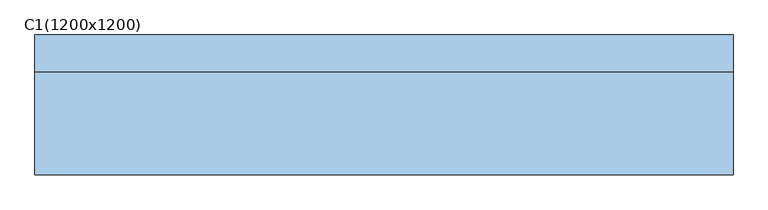
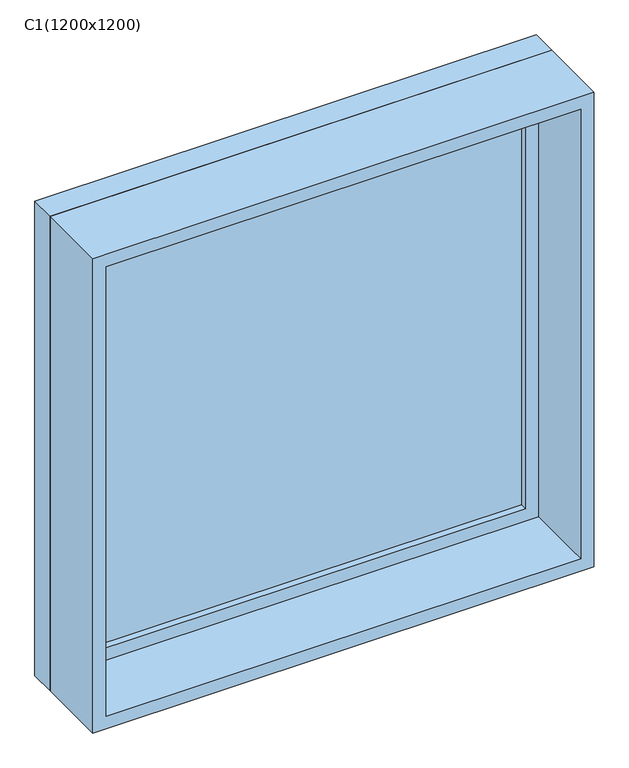
"""IFC4 building model written with IfcOpenShell, lengths in millimetres: window geometry, 固定窗 : C1(1200x1200)."""

import ifcopenshell
import ifcopenshell.guid

model = None  # the IFC model being written
_history = None  # IfcOwnerHistory: only IFC2X3 demands one
_inside = {}  # id of a spatial element -> (the spatial element, [elements in it])
_under = {}  # id of a project, library or spatial element -> (it, [spatial elements below it])
_declared = {}  # id of a project -> (the project, [libraries it declares])
_typed = {}  # id of a type object -> (the type object, [elements of that type])
_made_of = {}  # id of a material, layer set ... -> (it, [elements and type objects made of it])


def new_model(schema):
    """Start an empty IFC model of exactly this schema.

    Asked for "IFC4X3", IfcOpenShell would pick the latest addendum, in which some entities
    have other attributes; the version numbers below select the first issue.
    IFC2X3 requires an IfcOwnerHistory on every rooted entity: one is made here for all.
    """
    global model, _history
    if schema == "IFC4X3":
        model = ifcopenshell.file(schema_version=(4, 3, 0, 0))
    else:
        model = ifcopenshell.file(schema=schema)
    _inside.clear()
    _under.clear()
    _declared.clear()
    _typed.clear()
    _made_of.clear()
    _history = None
    if model.schema == "IFC2X3":
        org = make("IfcOrganization", Name="unknown")
        user = make(
            "IfcPersonAndOrganization",
            ThePerson=make("IfcPerson", FamilyName="unknown"),
            TheOrganization=org,
        )
        app = make(
            "IfcApplication",
            ApplicationDeveloper=org,
            Version="unknown",
            ApplicationFullName="unknown",
            ApplicationIdentifier="unknown",
        )
        _history = make(
            "IfcOwnerHistory",
            OwningUser=user,
            OwningApplication=app,
            ChangeAction="ADDED",
            CreationDate=0,
        )
    return model


def make(cls, **values):
    """One entity of the class cls with the attributes given. An attribute that is None is left unset."""
    return model.create_entity(
        cls, **{name: value for name, value in values.items() if value is not None}
    )


def rooted(cls, **values):
    """An entity with a GlobalId (a new one), such as an element, a storey or a relation."""
    return make(cls, GlobalId=ifcopenshell.guid.new(), OwnerHistory=_history, **values)


def si_unit(unit_type, name, prefix=None):
    """IfcSIUnit, for example si_unit("LENGTHUNIT", "METRE", prefix="MILLI")."""
    return make("IfcSIUnit", UnitType=unit_type, Prefix=prefix, Name=name)


def assignment(units):
    """IfcUnitAssignment: the units of a project."""
    return None if units is None else make("IfcUnitAssignment", Units=units)


def point(xyz):
    """IfcCartesianPoint."""
    return None if xyz is None else make("IfcCartesianPoint", Coordinates=xyz)


def direction(xyz):
    """IfcDirection."""
    return None if xyz is None else make("IfcDirection", DirectionRatios=xyz)


def frame(location, z_axis=None, x_axis=None):
    """IfcAxis2Placement3D, a coordinate frame: its origin and axes. An axis left out is left unset."""
    return make(
        "IfcAxis2Placement3D",
        Location=point(location),
        Axis=direction(z_axis),
        RefDirection=direction(x_axis),
    )


def origin():
    """The frame at (0, 0, 0) with its axes left unset."""
    return frame((0.0, 0.0, 0.0))


def place(relative_to, where):
    """IfcLocalPlacement: puts the frame where relative to a parent placement (None: the world)."""
    return make(
        "IfcLocalPlacement", PlacementRelTo=relative_to, RelativePlacement=where
    )


def context(
    kind, dimensions, precision=None, world=None, true_north=None, identifier=None
):
    """IfcGeometricRepresentationContext, for example the 3D "Model" context."""
    return make(
        "IfcGeometricRepresentationContext",
        ContextIdentifier=identifier,
        ContextType=kind,
        CoordinateSpaceDimension=dimensions,
        Precision=precision,
        WorldCoordinateSystem=world,
        TrueNorth=true_north,
    )


def project(units=None, contexts=None):
    """IfcProject with its units and contexts."""
    return rooted(
        "IfcProject",
        Name="project",
        RepresentationContexts=contexts,
        UnitsInContext=assignment(units),
    )


def spatial(cls, under=None, at=None, **own):
    """A site, building, storey or space (cls), placed at a placement, below another one or the project."""
    s = rooted(cls, ObjectPlacement=at, **own)
    if under is not None:
        _under.setdefault(under.id(), (under, []))[1].append(s)
    return s


def polyline(points):
    """IfcPolyline through the points."""
    return make("IfcPolyline", Points=[point(p) for p in points])


def outline(outer, holes=None, kind="AREA"):
    """IfcArbitraryClosedProfileDef: a profile drawn as a closed curve; with holes, ...WithVoids."""
    if holes is None:
        return make("IfcArbitraryClosedProfileDef", ProfileType=kind, OuterCurve=outer)
    return make(
        "IfcArbitraryProfileDefWithVoids",
        ProfileType=kind,
        OuterCurve=outer,
        InnerCurves=holes,
    )


def extrude(swept, where, along, depth):
    """IfcExtrudedAreaSolid: the profile swept, set in the frame where, extruded along a direction by depth."""
    return make(
        "IfcExtrudedAreaSolid",
        SweptArea=swept,
        Position=where,
        ExtrudedDirection=direction(along),
        Depth=depth,
    )


def shape(context_of_items, identifier, shape_type, items):
    """IfcShapeRepresentation: the items that make up one representation, for example the "Body"."""
    return make(
        "IfcShapeRepresentation",
        ContextOfItems=context_of_items,
        RepresentationIdentifier=identifier,
        RepresentationType=shape_type,
        Items=items,
    )


def source(mapping_origin, context_of_items, identifier, shape_type, items):
    """IfcRepresentationMap: a shape defined once, which mapped items show again and again."""
    return make(
        "IfcRepresentationMap",
        MappingOrigin=mapping_origin,
        MappedRepresentation=shape(context_of_items, identifier, shape_type, items),
    )


def transform(
    local_origin,
    x_axis=None,
    y_axis=None,
    z_axis=None,
    scale=None,
    scale2=None,
    scale3=None,
    uniform=True,
):
    """IfcCartesianTransformationOperator3D, or its non-uniform kind. x_axis, y_axis, z_axis: its Axis1, 2, 3."""
    if uniform:
        return make(
            "IfcCartesianTransformationOperator3D",
            Axis1=direction(x_axis),
            Axis2=direction(y_axis),
            LocalOrigin=point(local_origin),
            Scale=scale,
            Axis3=direction(z_axis),
        )
    return make(
        "IfcCartesianTransformationOperator3DnonUniform",
        Axis1=direction(x_axis),
        Axis2=direction(y_axis),
        LocalOrigin=point(local_origin),
        Scale=scale,
        Axis3=direction(z_axis),
        Scale2=scale2,
        Scale3=scale3,
    )


def mapped(mapping_source, mapping_target):
    """IfcMappedItem: shows the shape of a source again, moved by a transform."""
    return make(
        "IfcMappedItem", MappingSource=mapping_source, MappingTarget=mapping_target
    )


def made_of(thing, what):
    """Note that an element or type object is made of a material, layer set ...; save() writes the relation."""
    if what is not None:
        _made_of.setdefault(what.id(), (what, []))[1].append(thing)
    return thing


def element(
    cls,
    number,
    at=None,
    inside=None,
    cuts=None,
    type_object=None,
    material=None,
    context=None,
    identifier="Body",
    shape_type=None,
    held_by="IfcProductDefinitionShape",
    body=None,
    shapes=None,
    **own,
):
    """One element of the class cls, such as IfcWall. Its Tag is "e" and its number.

    at: its placement. inside: the storey or other place that contains it. cuts: it is an
    opening in that element (IfcRelVoidsElement). A single representation is given by context,
    identifier, shape_type and body (its items); several are given by shapes. held_by: the class
    of the entity that holds the representations. save() writes the other relations.
    """
    e = rooted(cls, Tag="e%d" % number, ObjectPlacement=at, **own)
    if body is not None:
        shapes = [shape(context, identifier, shape_type, body)]
    if shapes is not None:
        e.Representation = make(held_by, Representations=shapes)
    if inside is not None:
        _inside.setdefault(inside.id(), (inside, []))[1].append(e)
    if cuts is not None:
        rooted(
            "IfcRelVoidsElement", RelatingBuildingElement=cuts, RelatedOpeningElement=e
        )
    if type_object is not None:
        _typed.setdefault(type_object.id(), (type_object, []))[1].append(e)
    return made_of(e, material)


def aggregate(whole, parts):
    """IfcRelAggregates: a whole, such as a stair, and the parts it consists of."""
    return rooted("IfcRelAggregates", RelatingObject=whole, RelatedObjects=parts)


def save(model, path):
    """Write the relations noted so far, then the file.

    IfcRelAggregates (storeys below a building ...), IfcRelContainedInSpatialStructure (elements
    in a storey), IfcRelDefinesByType, IfcRelAssociatesMaterial and IfcRelDeclares: one each for
    every whole, place, type object, material and project.
    """
    for whole, parts in _under.values():
        aggregate(whole, parts)
    for where, things in _inside.values():
        rooted(
            "IfcRelContainedInSpatialStructure",
            RelatedElements=things,
            RelatingStructure=where,
        )
    for kind, things in _typed.values():
        rooted("IfcRelDefinesByType", RelatedObjects=things, RelatingType=kind)
    for what, things in _made_of.values():
        rooted("IfcRelAssociatesMaterial", RelatedObjects=things, RelatingMaterial=what)
    for by, libraries in _declared.values():
        rooted("IfcRelDeclares", RelatingContext=by, RelatedDefinitions=libraries)
    model.write(path)


def c1_1200x1200_024adce4(model_context):
    return source(origin(), model_context, "Body", "SweptSolid", [
        extrude(outline(polyline([(498.4, 71.425), (-574.6, 71.425), (-574.6, 84.125), (498.4, 84.125), (498.4, 71.425)])), frame((0.0, 0.0, 963.5), z_axis=(0.0, 0.0, 1.0), x_axis=(1.0, 0.0, 0.0)), (0.0, 0.0, 1.0), 1073.0),
        extrude(outline(polyline([(2080.95, -619.05), (919.05, -619.05), (919.05, 542.85), (2080.95, 542.85), (2080.95, -619.05)]), holes=[polyline([(2036.5, -574.6), (2036.5, 498.4), (963.5, 498.4), (963.5, -574.6), (2036.5, -574.6)])]), frame((0.0, 55.55, 0.0), z_axis=(0.0, 1.0, 0.0), x_axis=(0.0, 0.0, 1.0)), (0.0, 0.0, 1.0), 44.45),
        extrude(outline(polyline([(2100.0, -638.1), (900.0, -638.1), (900.0, 561.9), (2100.0, 561.9), (2100.0, -638.1)]), holes=[polyline([(2068.25, -606.35), (2068.25, 530.15), (931.75, 530.15), (931.75, -606.35), (2068.25, -606.35)])]), frame((0.0, -120.0, 0.0), z_axis=(0.0, 1.0, 0.0), x_axis=(0.0, 0.0, 1.0)), (0.0, 0.0, 1.0), 175.55),
        extrude(outline(polyline([(2100.0, 561.9), (2100.0, -638.1), (900.0, -638.1), (900.0, 561.9), (2100.0, 561.9)]), holes=[polyline([(2080.95, 542.85), (919.05, 542.85), (919.05, -619.05), (2080.95, -619.05), (2080.95, 542.85)])]), frame((0.0, 55.55, 0.0), z_axis=(0.0, 1.0, 0.0), x_axis=(0.0, 0.0, 1.0)), (0.0, 0.0, 1.0), 64.45),
    ])


if __name__ == "__main__":
    model = new_model("IFC4")
    model_context = context("Model", 3, world=origin())
    ifc_project = project(units=[si_unit("LENGTHUNIT", "METRE", prefix="MILLI")], contexts=[model_context])
    site = spatial("IfcSite", under=ifc_project)
    building = spatial("IfcBuilding", under=site)
    placement = place(None, origin())
    c1_1200x1200_shape = c1_1200x1200_024adce4(model_context)
    element("IfcWindow", 1, ObjectType="固定窗 : C1(1200x1200)", at=placement, inside=building, context=model_context, shape_type="MappedRepresentation", body=[
        mapped(c1_1200x1200_shape, transform((0.0, 0.0, 0.0), x_axis=(1.0, 0.0, 0.0), y_axis=(0.0, 1.0, 0.0), z_axis=(0.0, 0.0, 1.0))),
    ])
    save(model, "model.ifc")

# Revit data of these elements
# Project information
#   项目发布日期 = "出图日期"
#   项目状态 = "项目状态"
#   客户姓名 = "所有者"
#   项目地址 = "请在此处输入地址"
#   项目名称 = "项目名称"
#   项目编号 = "项目编号"
# Type "固定窗 : C1(1200x1200)"
#   Type Mark = "C1518"
#   Construction Type Id = "SGL"
#   Analytic Construction = "大型单层玻璃窗"
#   Visual Light Transmittance = 0.9
#   Solar Heat Gain Coefficient = 0.86
#   Rough Width = 1200 mm
#   Rough Height = 1200 mm
#   Heat Transfer Coefficient (U) = 5.5617 W/(m²·K)
#   Height = 1200 mm
#   默认窗台高度 = 900 mm
#   Width = 1200 mm
#   窗嵌入 = 20 mm
#   高窗平面 [instance default] = no
#   通用窗平面 [instance default] = yes
#   玻璃 = none
#   框架材质 = none
#   Wall Closure = (empty or 0)
# Element 1 (IfcWindow, "固定窗 : C1(1200x1200)")
#   Materials on its faces: "玻璃"
# Materials
#   "玻璃": class "玻璃", colour RGB 0 128 192, transparency 0.9, Description = "钠钙玻璃", Cost = 0
